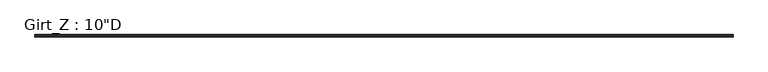
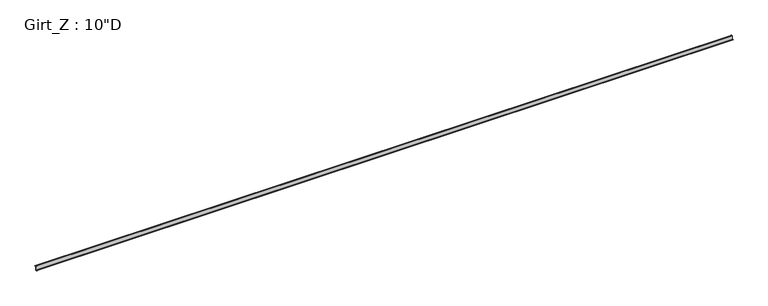
"""IFC4 building model written with IfcOpenShell, lengths in millimetres: beam geometry."""

from ifc_helpers import new_model, si_unit, point, frame, frame_2d, origin, place, context, project, spatial, polyline, circle_curve, trimmed, segment, composite_curve, outline, extrude, source, transform, mapped, element, save


def beam_fa991611(model_context):
    return source(origin(), model_context, "Body", "SweptSolid", [
        extrude(outline(composite_curve([segment(polyline([(63.5, 127.0), (75.745104, 112.4068534), (73.6169367, 110.621109), (62.204539, 124.221875), (3.3005807, 124.221875)]), True, "CONTINUOUS"), segment(trimmed(circle_curve(frame_2d((3.3741066, 122.2381931)), 1.9850441), [point((3.3005807, 124.221875))], [point((1.3890625, 122.2381931))], True, "CARTESIAN"), True, "CONTINUOUS"), segment(polyline([(1.3890625, 122.2381931), (1.3890625, -122.2375)]), True, "CONTINUOUS"), segment(trimmed(circle_curve(frame_2d((-3.3734375, -122.2375)), 4.7625), [point((1.3890625, -122.2375))], [point((-3.3734375, -127.0))], False, "CARTESIAN"), True, "CONTINUOUS"), segment(polyline([(-3.3734375, -127.0), (-63.5, -127.0), (-75.745104, -112.4068534), (-73.6169367, -110.621109), (-62.204539, -124.221875), (-3.2694106, -124.221875)]), True, "CONTINUOUS"), segment(trimmed(circle_curve(frame_2d((-3.3748024, -122.2389339)), 1.9857399), [point((-3.2694106, -124.221875))], [point((-1.3890625, -122.2389339))], True, "CARTESIAN"), True, "CONTINUOUS"), segment(polyline([(-1.3890625, -122.2389339), (-1.3890625, 122.2375)]), True, "CONTINUOUS"), segment(trimmed(circle_curve(frame_2d((3.3734375, 122.2375)), 4.7625), [point((-1.3890625, 122.2375))], [point((3.3734375, 127.0))], False, "CARTESIAN"), True, "CONTINUOUS"), segment(polyline([(3.3734375, 127.0), (63.5, 127.0)]), True, "CONTINUOUS")], self_intersect=False)), frame((-22098.0, 0.0, 0.0), z_axis=(1.0, 0.0, 0.0), x_axis=(0.0, 1.0, 0.0)), (0.0, 0.0, 1.0), 44107.1),
    ])


if __name__ == "__main__":
    model = new_model("IFC4")
    model_context = context("Model", 3, world=origin())
    ifc_project = project(units=[si_unit("LENGTHUNIT", "METRE", prefix="MILLI")], contexts=[model_context])
    site = spatial("IfcSite", under=ifc_project)
    building = spatial("IfcBuilding", under=site)
    placement = place(None, origin())
    beam_shape = beam_fa991611(model_context)
    element("IfcBeam", 1, ObjectType="Girt_Z : 10\"D", at=placement, inside=building, context=model_context, shape_type="MappedRepresentation", body=[
        mapped(beam_shape, transform((0.0, 0.0, 0.0), x_axis=(1.0, 0.0, 0.0), y_axis=(0.0, 1.0, 0.0), z_axis=(0.0, 0.0, 1.0))),
    ])
    save(model, "model.ifc")

# Revit data of these elements
# Type "Girt_Z : 10\"D"
#   Web_Thickness = 0' - 0 7/64"
#   Length [instance default] = 10' - 0"
#   Leg_1 = 0' - 2 1/2"
#   Height = 0' - 10"
